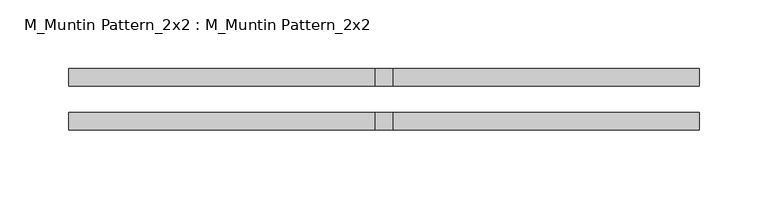
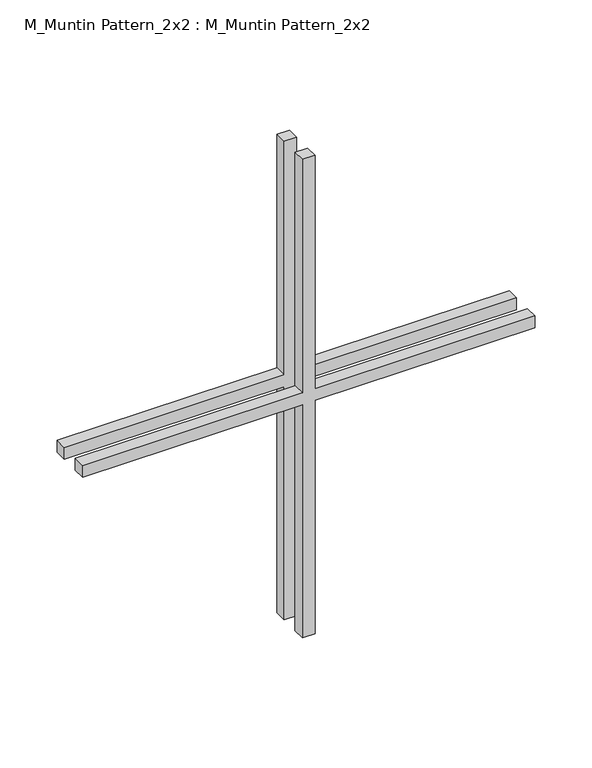
"""IFC4 building model written with IfcOpenShell, lengths in millimetres: proxy geometry, M_Muntin Pattern_2x2 : M_Muntin Pattern_2x2."""

from ifc_helpers import new_model, si_unit, frame, origin, place, context, project, spatial, polyline, outline, extrude, source, transform, mapped, element, save


def m_muntin_pattern_2x2_m_muntin_pattern_2x2_e9cb9308(model_context):
    return source(origin(), model_context, "Body", "SweptSolid", [
        extrude(outline(polyline([(261.9375, -6.35), (261.9375, -228.6), (249.2375, -228.6), (249.2375, -6.35), (0.0, -6.35), (0.0, 6.35), (249.2375, 6.35), (249.2375, 228.6), (261.9375, 228.6), (261.9375, 6.35), (511.175, 6.35), (511.175, -6.35), (261.9375, -6.35)])), frame((0.0, -22.225, 0.0), z_axis=(0.0, 1.0, 0.0), x_axis=(0.0, 0.0, 1.0)), (0.0, 0.0, 1.0), 12.7),
        extrude(outline(polyline([(261.9375, -6.35), (261.9375, -228.6), (249.2375, -228.6), (249.2375, -6.35), (0.0, -6.35), (0.0, 6.35), (249.2375, 6.35), (249.2375, 228.6), (261.9375, 228.6), (261.9375, 6.35), (511.175, 6.35), (511.175, -6.35), (261.9375, -6.35)])), frame((0.0, 9.525, 0.0), z_axis=(0.0, 1.0, 0.0), x_axis=(0.0, 0.0, 1.0)), (0.0, 0.0, 1.0), 12.7),
    ])


if __name__ == "__main__":
    model = new_model("IFC4")
    model_context = context("Model", 3, world=origin())
    ifc_project = project(units=[si_unit("LENGTHUNIT", "METRE", prefix="MILLI")], contexts=[model_context])
    site = spatial("IfcSite", under=ifc_project)
    building = spatial("IfcBuilding", under=site)
    placement = place(None, origin())
    m_muntin_pattern_2x2_m_muntin_pattern_2x2_shape = m_muntin_pattern_2x2_m_muntin_pattern_2x2_e9cb9308(model_context)
    element("IfcBuildingElementProxy", 1, Name="M_Muntin Pattern_2x2 : M_Muntin Pattern_2x2", ObjectType="M_Muntin Pattern_2x2 : M_Muntin Pattern_2x2", at=placement, inside=building, context=model_context, shape_type="MappedRepresentation", body=[
        mapped(m_muntin_pattern_2x2_m_muntin_pattern_2x2_shape, transform((0.0, 0.0, 0.0), x_axis=(1.0, 0.0, 0.0), y_axis=(0.0, 1.0, 0.0), z_axis=(0.0, 0.0, 1.0))),
    ])
    save(model, "model.ifc")

# Revit data of these elements
# Type "M_Muntin Pattern_2x2 : M_Muntin Pattern_2x2"
#   Width [instance default] = 3' - 11.24409"
#   Thickness = 0' - 0 1/2"
#   Height [instance default] = 3' - 11.24409"
#   Distance = 0' - 0 3/4"
#   Interior Material [instance default] = none
#   Exterior Material [instance default] = none
#   Default Elevation = 0
# Element 1 (IfcBuildingElementProxy, "M_Muntin Pattern_2x2 : M_Muntin Pattern_2x2")
#   Width = 1' - 6"
#   Height = 1' - 8 1/8"
#   Interior Material = Wood - Stained
#   Exterior Material = Clad - White
#   Materials on its faces: "Clad - White", "Wood - Stained"
# Materials
#   "Clad - White": class "Wood", colour RGB 242 242 238, transparency 0, Cost = 0
#   "Wood - Stained": class "Wood", colour RGB 224 178 126, transparency 0, Cost = 0
